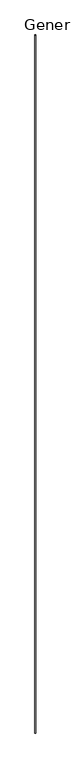
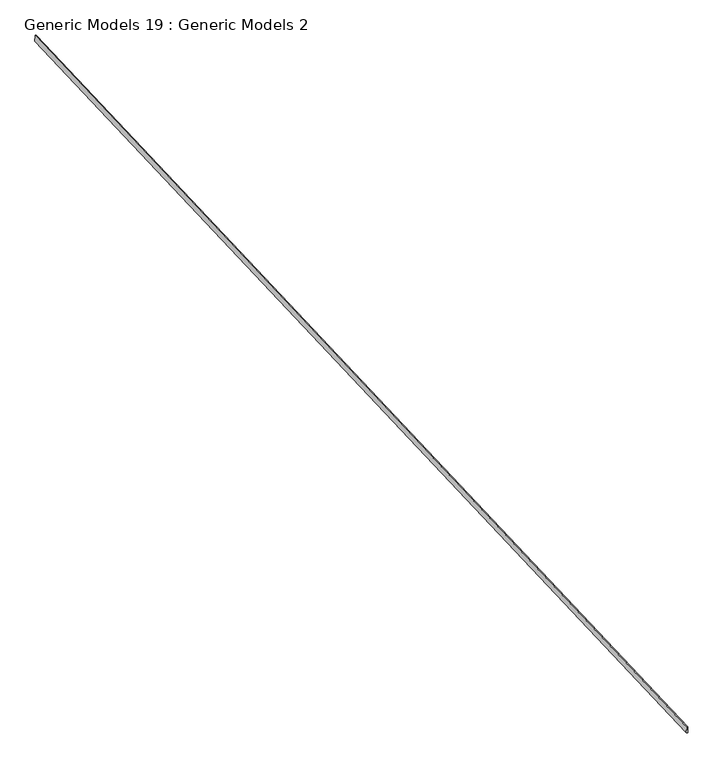
"""IFC4 building model written with IfcOpenShell, lengths in millimetres: proxy geometry, Generic Models 19 : Generic Models 2."""

from ifc_helpers import new_model, si_unit, frame, origin, place, context, project, spatial, polyline, outline, extrude, source, transform, mapped, element, save


def generic_models_19_generic_models_2_17a90d81(model_context):
    return source(origin(), model_context, "Body", "SweptSolid", [
        extrude(outline(polyline([(0.0, -38.1), (0.0, 0.0), (33406.7702703, 0.0), (33406.7702703, -38.1), (0.0, -38.1)])), frame((667506.057152, -569967.3099899, 8444.8338132), z_axis=(0.0, -0.04163054471217683, 0.9991330730923521), x_axis=(0.0, 0.9991330730923521, 0.04163054471217683)), (0.0, 0.0, 1.0), 184.15),
    ])


if __name__ == "__main__":
    model = new_model("IFC4")
    model_context = context("Model", 3, world=origin())
    ifc_project = project(units=[si_unit("LENGTHUNIT", "METRE", prefix="MILLI")], contexts=[model_context])
    site = spatial("IfcSite", under=ifc_project)
    building = spatial("IfcBuilding", under=site)
    placement = place(None, origin())
    generic_models_19_generic_models_2_shape = generic_models_19_generic_models_2_17a90d81(model_context)
    element("IfcBuildingElementProxy", 1, Name="Generic Models 19 : Generic Models 2", ObjectType="Generic Models 19 : Generic Models 2", at=placement, inside=building, context=model_context, shape_type="MappedRepresentation", body=[
        mapped(generic_models_19_generic_models_2_shape, transform((0.0, 0.0, 0.0), x_axis=(1.0, 0.0, 0.0), y_axis=(0.0, 1.0, 0.0), z_axis=(0.0, 0.0, 1.0))),
    ])
    save(model, "model.ifc")

# Revit data of these elements
# Element 1 (IfcBuildingElementProxy, "Generic Models 19 : Generic Models 2")
#   Materials on its faces: "FIRE RETARDTANT WOOD BLOCKING - SIZE AS NEC."
# Materials
#   "FIRE RETARDTANT WOOD BLOCKING - SIZE AS NEC.": class "Wood", colour RGB 144 113 62, transparency 0, Description = "Pinus Echinata", Cost = 0
